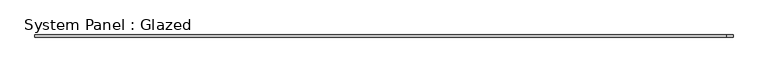
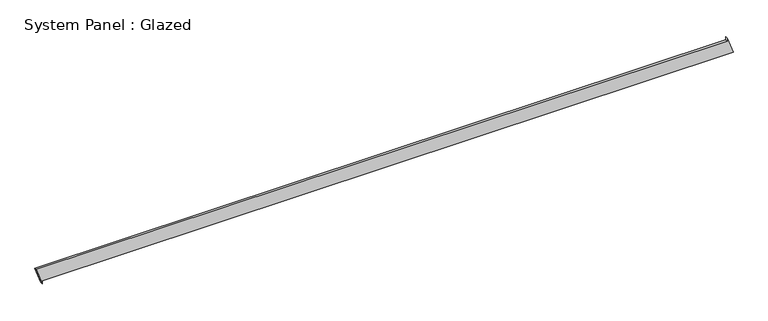
"""IFC4 building model written with IfcOpenShell, lengths in millimetres: plate geometry, System Panel : Glazed."""

import ifcopenshell
import ifcopenshell.guid

model = None  # the IFC model being written
_history = None  # IfcOwnerHistory: only IFC2X3 demands one
_inside = {}  # id of a spatial element -> (the spatial element, [elements in it])
_under = {}  # id of a project, library or spatial element -> (it, [spatial elements below it])
_declared = {}  # id of a project -> (the project, [libraries it declares])
_typed = {}  # id of a type object -> (the type object, [elements of that type])
_made_of = {}  # id of a material, layer set ... -> (it, [elements and type objects made of it])


def new_model(schema):
    """Start an empty IFC model of exactly this schema.

    Asked for "IFC4X3", IfcOpenShell would pick the latest addendum, in which some entities
    have other attributes; the version numbers below select the first issue.
    IFC2X3 requires an IfcOwnerHistory on every rooted entity: one is made here for all.
    """
    global model, _history
    if schema == "IFC4X3":
        model = ifcopenshell.file(schema_version=(4, 3, 0, 0))
    else:
        model = ifcopenshell.file(schema=schema)
    _inside.clear()
    _under.clear()
    _declared.clear()
    _typed.clear()
    _made_of.clear()
    _history = None
    if model.schema == "IFC2X3":
        org = make("IfcOrganization", Name="unknown")
        user = make(
            "IfcPersonAndOrganization",
            ThePerson=make("IfcPerson", FamilyName="unknown"),
            TheOrganization=org,
        )
        app = make(
            "IfcApplication",
            ApplicationDeveloper=org,
            Version="unknown",
            ApplicationFullName="unknown",
            ApplicationIdentifier="unknown",
        )
        _history = make(
            "IfcOwnerHistory",
            OwningUser=user,
            OwningApplication=app,
            ChangeAction="ADDED",
            CreationDate=0,
        )
    return model


def make(cls, **values):
    """One entity of the class cls with the attributes given. An attribute that is None is left unset."""
    return model.create_entity(
        cls, **{name: value for name, value in values.items() if value is not None}
    )


def rooted(cls, **values):
    """An entity with a GlobalId (a new one), such as an element, a storey or a relation."""
    return make(cls, GlobalId=ifcopenshell.guid.new(), OwnerHistory=_history, **values)


def si_unit(unit_type, name, prefix=None):
    """IfcSIUnit, for example si_unit("LENGTHUNIT", "METRE", prefix="MILLI")."""
    return make("IfcSIUnit", UnitType=unit_type, Prefix=prefix, Name=name)


def assignment(units):
    """IfcUnitAssignment: the units of a project."""
    return None if units is None else make("IfcUnitAssignment", Units=units)


def point(xyz):
    """IfcCartesianPoint."""
    return None if xyz is None else make("IfcCartesianPoint", Coordinates=xyz)


def direction(xyz):
    """IfcDirection."""
    return None if xyz is None else make("IfcDirection", DirectionRatios=xyz)


def frame(location, z_axis=None, x_axis=None):
    """IfcAxis2Placement3D, a coordinate frame: its origin and axes. An axis left out is left unset."""
    return make(
        "IfcAxis2Placement3D",
        Location=point(location),
        Axis=direction(z_axis),
        RefDirection=direction(x_axis),
    )


def origin():
    """The frame at (0, 0, 0) with its axes left unset."""
    return frame((0.0, 0.0, 0.0))


def place(relative_to, where):
    """IfcLocalPlacement: puts the frame where relative to a parent placement (None: the world)."""
    return make(
        "IfcLocalPlacement", PlacementRelTo=relative_to, RelativePlacement=where
    )


def context(
    kind, dimensions, precision=None, world=None, true_north=None, identifier=None
):
    """IfcGeometricRepresentationContext, for example the 3D "Model" context."""
    return make(
        "IfcGeometricRepresentationContext",
        ContextIdentifier=identifier,
        ContextType=kind,
        CoordinateSpaceDimension=dimensions,
        Precision=precision,
        WorldCoordinateSystem=world,
        TrueNorth=true_north,
    )


def project(units=None, contexts=None):
    """IfcProject with its units and contexts."""
    return rooted(
        "IfcProject",
        Name="project",
        RepresentationContexts=contexts,
        UnitsInContext=assignment(units),
    )


def spatial(cls, under=None, at=None, **own):
    """A site, building, storey or space (cls), placed at a placement, below another one or the project."""
    s = rooted(cls, ObjectPlacement=at, **own)
    if under is not None:
        _under.setdefault(under.id(), (under, []))[1].append(s)
    return s


def polyline(points):
    """IfcPolyline through the points."""
    return make("IfcPolyline", Points=[point(p) for p in points])


def outline(outer, holes=None, kind="AREA"):
    """IfcArbitraryClosedProfileDef: a profile drawn as a closed curve; with holes, ...WithVoids."""
    if holes is None:
        return make("IfcArbitraryClosedProfileDef", ProfileType=kind, OuterCurve=outer)
    return make(
        "IfcArbitraryProfileDefWithVoids",
        ProfileType=kind,
        OuterCurve=outer,
        InnerCurves=holes,
    )


def extrude(swept, where, along, depth):
    """IfcExtrudedAreaSolid: the profile swept, set in the frame where, extruded along a direction by depth."""
    return make(
        "IfcExtrudedAreaSolid",
        SweptArea=swept,
        Position=where,
        ExtrudedDirection=direction(along),
        Depth=depth,
    )


def shape(context_of_items, identifier, shape_type, items):
    """IfcShapeRepresentation: the items that make up one representation, for example the "Body"."""
    return make(
        "IfcShapeRepresentation",
        ContextOfItems=context_of_items,
        RepresentationIdentifier=identifier,
        RepresentationType=shape_type,
        Items=items,
    )


def source(mapping_origin, context_of_items, identifier, shape_type, items):
    """IfcRepresentationMap: a shape defined once, which mapped items show again and again."""
    return make(
        "IfcRepresentationMap",
        MappingOrigin=mapping_origin,
        MappedRepresentation=shape(context_of_items, identifier, shape_type, items),
    )


def transform(
    local_origin,
    x_axis=None,
    y_axis=None,
    z_axis=None,
    scale=None,
    scale2=None,
    scale3=None,
    uniform=True,
):
    """IfcCartesianTransformationOperator3D, or its non-uniform kind. x_axis, y_axis, z_axis: its Axis1, 2, 3."""
    if uniform:
        return make(
            "IfcCartesianTransformationOperator3D",
            Axis1=direction(x_axis),
            Axis2=direction(y_axis),
            LocalOrigin=point(local_origin),
            Scale=scale,
            Axis3=direction(z_axis),
        )
    return make(
        "IfcCartesianTransformationOperator3DnonUniform",
        Axis1=direction(x_axis),
        Axis2=direction(y_axis),
        LocalOrigin=point(local_origin),
        Scale=scale,
        Axis3=direction(z_axis),
        Scale2=scale2,
        Scale3=scale3,
    )


def mapped(mapping_source, mapping_target):
    """IfcMappedItem: shows the shape of a source again, moved by a transform."""
    return make(
        "IfcMappedItem", MappingSource=mapping_source, MappingTarget=mapping_target
    )


def made_of(thing, what):
    """Note that an element or type object is made of a material, layer set ...; save() writes the relation."""
    if what is not None:
        _made_of.setdefault(what.id(), (what, []))[1].append(thing)
    return thing


def element(
    cls,
    number,
    at=None,
    inside=None,
    cuts=None,
    type_object=None,
    material=None,
    context=None,
    identifier="Body",
    shape_type=None,
    held_by="IfcProductDefinitionShape",
    body=None,
    shapes=None,
    **own,
):
    """One element of the class cls, such as IfcWall. Its Tag is "e" and its number.

    at: its placement. inside: the storey or other place that contains it. cuts: it is an
    opening in that element (IfcRelVoidsElement). A single representation is given by context,
    identifier, shape_type and body (its items); several are given by shapes. held_by: the class
    of the entity that holds the representations. save() writes the other relations.
    """
    e = rooted(cls, Tag="e%d" % number, ObjectPlacement=at, **own)
    if body is not None:
        shapes = [shape(context, identifier, shape_type, body)]
    if shapes is not None:
        e.Representation = make(held_by, Representations=shapes)
    if inside is not None:
        _inside.setdefault(inside.id(), (inside, []))[1].append(e)
    if cuts is not None:
        rooted(
            "IfcRelVoidsElement", RelatingBuildingElement=cuts, RelatedOpeningElement=e
        )
    if type_object is not None:
        _typed.setdefault(type_object.id(), (type_object, []))[1].append(e)
    return made_of(e, material)


def aggregate(whole, parts):
    """IfcRelAggregates: a whole, such as a stair, and the parts it consists of."""
    return rooted("IfcRelAggregates", RelatingObject=whole, RelatedObjects=parts)


def save(model, path):
    """Write the relations noted so far, then the file.

    IfcRelAggregates (storeys below a building ...), IfcRelContainedInSpatialStructure (elements
    in a storey), IfcRelDefinesByType, IfcRelAssociatesMaterial and IfcRelDeclares: one each for
    every whole, place, type object, material and project.
    """
    for whole, parts in _under.values():
        aggregate(whole, parts)
    for where, things in _inside.values():
        rooted(
            "IfcRelContainedInSpatialStructure",
            RelatedElements=things,
            RelatingStructure=where,
        )
    for kind, things in _typed.values():
        rooted("IfcRelDefinesByType", RelatedObjects=things, RelatingType=kind)
    for what, things in _made_of.values():
        rooted("IfcRelAssociatesMaterial", RelatedObjects=things, RelatingMaterial=what)
    for by, libraries in _declared.values():
        rooted("IfcRelDeclares", RelatingContext=by, RelatedDefinitions=libraries)
    model.write(path)


def system_panel_glazed_fe5ea76c(model_context):
    return source(origin(), model_context, "Body", "SweptSolid", [
        extrude(outline(polyline([(0.0, -3956.7629895), (35.3553391, -3956.7629895), (35.3553391, 4027.1398136), (235.0472205, 3956.767991), (199.6918814, 3956.7680004), (199.6897639, -4027.1398136), (0.0, -3956.7629895)])), frame((0.0, -49.5, 0.0), z_axis=(0.0, 1.0, 0.0), x_axis=(0.0, 0.0, 1.0)), (0.0, 0.0, 1.0), 25.0),
    ])


if __name__ == "__main__":
    model = new_model("IFC4")
    model_context = context("Model", 3, world=origin())
    ifc_project = project(units=[si_unit("LENGTHUNIT", "METRE", prefix="MILLI")], contexts=[model_context])
    site = spatial("IfcSite", under=ifc_project)
    building = spatial("IfcBuilding", under=site)
    placement = place(None, origin())
    system_panel_glazed_shape = system_panel_glazed_fe5ea76c(model_context)
    element("IfcPlate", 1, ObjectType="System Panel : Glazed", at=placement, inside=building, context=model_context, shape_type="MappedRepresentation", body=[
        mapped(system_panel_glazed_shape, transform((0.0, 0.0, 0.0), x_axis=(1.0, 0.0, 0.0), y_axis=(0.0, 1.0, 0.0), z_axis=(0.0, 0.0, 1.0))),
    ])
    save(model, "model.ifc")

# Revit data of these elements
# Element 1 (IfcPlate, "System Panel : Glazed")
#   Materials on its faces: "Glass"
# Materials
#   "Glass": class "Glass", colour RGB 218 227 224, transparency 0.85, Description = "Soda Lime Glass", Cost = 0
